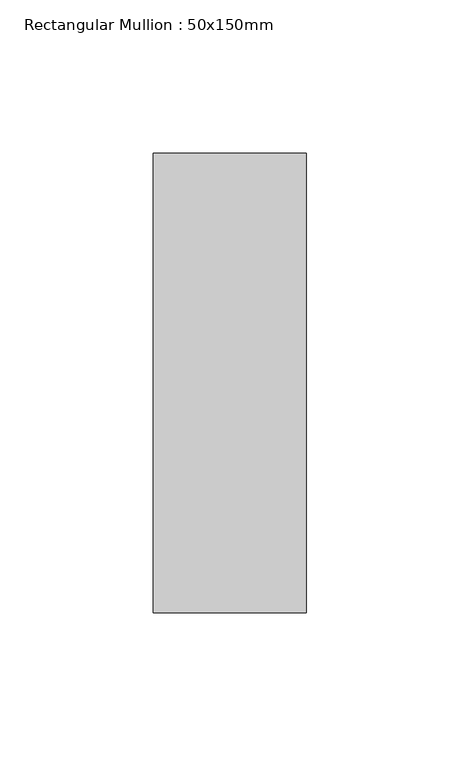
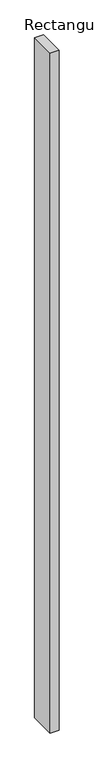
"""IFC4 building model written with IfcOpenShell, lengths in millimetres: member geometry, Rectangular Mullion : 50x150mm."""

from ifc_helpers import new_model, si_unit, frame, origin, place, context, project, spatial, polyline, outline, extrude, source, transform, mapped, element, save


def rectangular_mullion_50x150mm_1b9437d6(model_context):
    return source(origin(), model_context, "Body", "SweptSolid", [
        extrude(outline(polyline([(25.0, 75.0), (25.0, -75.0), (-25.0, -75.0), (-25.0, 75.0), (25.0, 75.0)])), frame((0.0, 0.0, -4000.0), z_axis=(0.0, 0.0, 1.0), x_axis=(1.0, 0.0, 0.0)), (0.0, 0.0, 1.0), 4000.0),
    ])


if __name__ == "__main__":
    model = new_model("IFC4")
    model_context = context("Model", 3, world=origin())
    ifc_project = project(units=[si_unit("LENGTHUNIT", "METRE", prefix="MILLI")], contexts=[model_context])
    site = spatial("IfcSite", under=ifc_project)
    building = spatial("IfcBuilding", under=site)
    placement = place(None, origin())
    rectangular_mullion_50x150mm_shape = rectangular_mullion_50x150mm_1b9437d6(model_context)
    element("IfcMember", 1, ObjectType="Rectangular Mullion : 50x150mm", at=placement, inside=building, context=model_context, shape_type="MappedRepresentation", body=[
        mapped(rectangular_mullion_50x150mm_shape, transform((0.0, 0.0, 0.0), x_axis=(1.0, 0.0, 0.0), y_axis=(0.0, 1.0, 0.0), z_axis=(0.0, 0.0, 1.0))),
    ])
    save(model, "model.ifc")

# Revit data of these elements
# Type "Rectangular Mullion : 50x150mm"
#   Keynote = "H11"
#   built-in parameter 1007304 = 0.492126 (stored number, unit not read)
#   built-in parameter 1007301 = 0.082021 (stored number, unit not read)
#   built-in parameter 1007300 = 0.082021 (stored number, unit not read)
# Element 1 (IfcMember, "Rectangular Mullion : 50x150mm")
#   Materials on its faces: "Aluminium"
# Materials
#   "Aluminium": class "Metal", colour RGB 247 247 247, transparency 0, Description = "Aluminium 6061", Cost = 0
